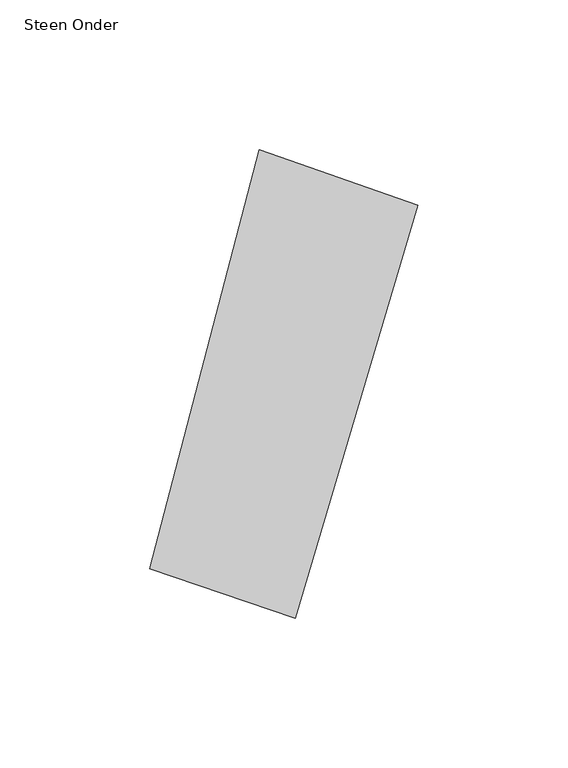
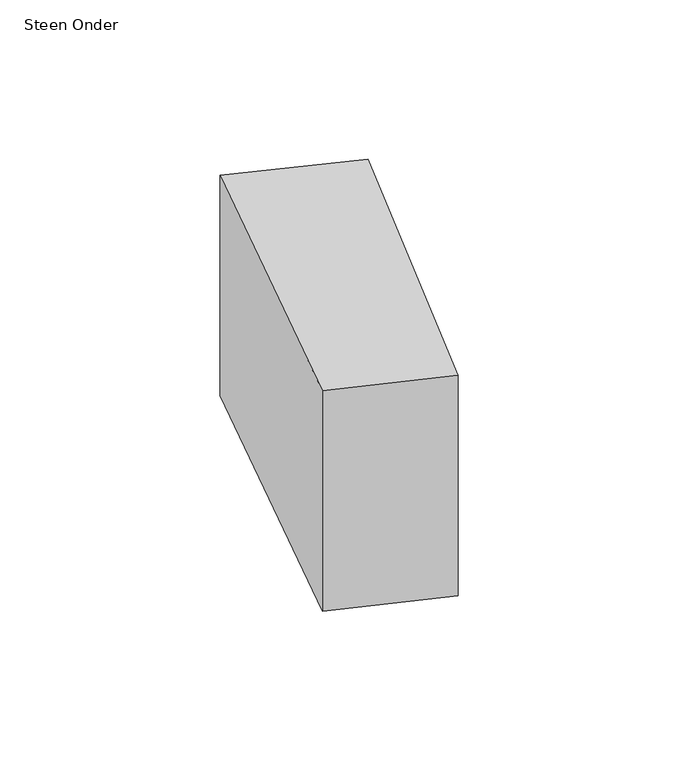
"""IFC4 building model written with IfcOpenShell, lengths in millimetres: proxy geometry, 00_GMA_steen_versie_4 : Steen Onder."""

from ifc_helpers import new_model, si_unit, origin, origin_with_axes, place, context, project, spatial, polyline, outline, extrude, source, transform, mapped, element, save


def steen_onder_c1beca46(model_context):
    return source(origin(), model_context, "Body", "SweptSolid", [
        extrude(outline(polyline([(120.6133537, 136.7972027), (79.6527434, -1.0277839), (31.1030604, 15.5240967), (67.7513793, 155.4133903), (120.6133537, 136.7972027)])), origin_with_axes(), (0.0, 0.0, 1.0), 100.0),
    ])


if __name__ == "__main__":
    model = new_model("IFC4")
    model_context = context("Model", 3, world=origin())
    ifc_project = project(units=[si_unit("LENGTHUNIT", "METRE", prefix="MILLI")], contexts=[model_context])
    site = spatial("IfcSite", under=ifc_project)
    building = spatial("IfcBuilding", under=site)
    placement = place(None, origin())
    steen_onder_shape = steen_onder_c1beca46(model_context)
    element("IfcBuildingElementProxy", 1, Name="00_GMA_steen_versie_4 : Steen Onder", ObjectType="00_GMA_steen_versie_4 : Steen Onder", at=placement, inside=building, context=model_context, shape_type="MappedRepresentation", body=[
        mapped(steen_onder_shape, transform((0.0, 0.0, 0.0), x_axis=(1.0, 0.0, 0.0), y_axis=(0.0, 1.0, 0.0), z_axis=(0.0, 0.0, 1.0))),
    ])
    save(model, "model.ifc")

# Revit data of these elements
# Type "00_GMA_steen_versie_4 : Steen Onder"
#   StootVoegHalfBoven [instance default] = 5 mm
#   StootVoegHalf [instance default] = 5 mm
#   StootVoegBreedteOnder = 10 mm
#   StootVoegBreedteBoven = 10 mm
#   Steendikte = 100 mm
#   LintVoegOnderHalf = 0 mm
#   LintVoegOnder = 0 mm
#   LintVoegBovenHalf = 5 mm
#   LintVoegBoven = 10 mm
#   materiaal = none
#   MateriaalVoeg = none
#   Default Elevation = 0
